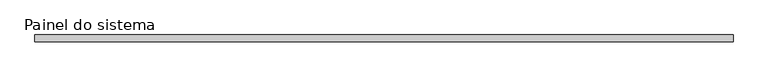
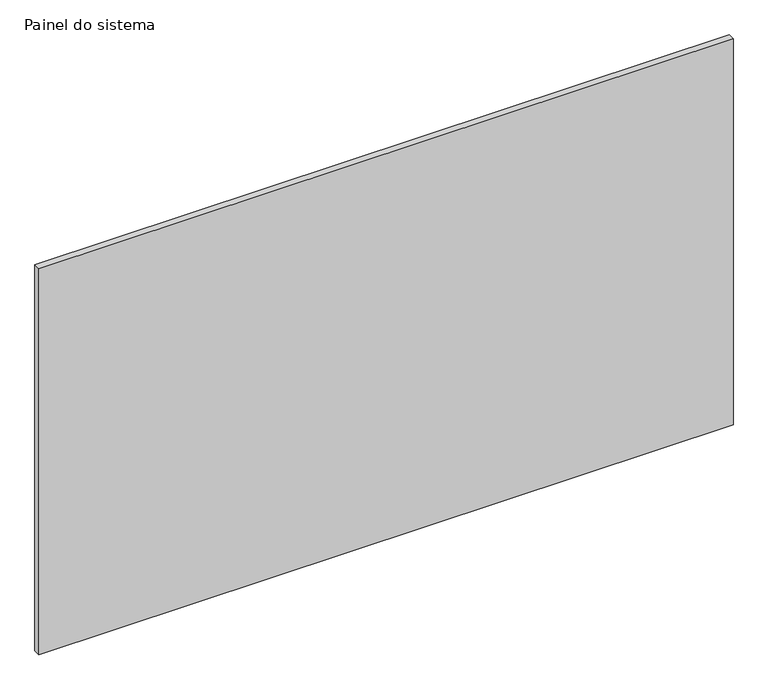
"""IFC4 building model written with IfcOpenShell, lengths in millimetres: plate geometry, Painel do sistema : Envidraçado."""

import ifcopenshell
import ifcopenshell.guid

model = None  # the IFC model being written
_history = None  # IfcOwnerHistory: only IFC2X3 demands one
_inside = {}  # id of a spatial element -> (the spatial element, [elements in it])
_under = {}  # id of a project, library or spatial element -> (it, [spatial elements below it])
_declared = {}  # id of a project -> (the project, [libraries it declares])
_typed = {}  # id of a type object -> (the type object, [elements of that type])
_made_of = {}  # id of a material, layer set ... -> (it, [elements and type objects made of it])


def new_model(schema):
    """Start an empty IFC model of exactly this schema.

    Asked for "IFC4X3", IfcOpenShell would pick the latest addendum, in which some entities
    have other attributes; the version numbers below select the first issue.
    IFC2X3 requires an IfcOwnerHistory on every rooted entity: one is made here for all.
    """
    global model, _history
    if schema == "IFC4X3":
        model = ifcopenshell.file(schema_version=(4, 3, 0, 0))
    else:
        model = ifcopenshell.file(schema=schema)
    _inside.clear()
    _under.clear()
    _declared.clear()
    _typed.clear()
    _made_of.clear()
    _history = None
    if model.schema == "IFC2X3":
        org = make("IfcOrganization", Name="unknown")
        user = make(
            "IfcPersonAndOrganization",
            ThePerson=make("IfcPerson", FamilyName="unknown"),
            TheOrganization=org,
        )
        app = make(
            "IfcApplication",
            ApplicationDeveloper=org,
            Version="unknown",
            ApplicationFullName="unknown",
            ApplicationIdentifier="unknown",
        )
        _history = make(
            "IfcOwnerHistory",
            OwningUser=user,
            OwningApplication=app,
            ChangeAction="ADDED",
            CreationDate=0,
        )
    return model


def make(cls, **values):
    """One entity of the class cls with the attributes given. An attribute that is None is left unset."""
    return model.create_entity(
        cls, **{name: value for name, value in values.items() if value is not None}
    )


def rooted(cls, **values):
    """An entity with a GlobalId (a new one), such as an element, a storey or a relation."""
    return make(cls, GlobalId=ifcopenshell.guid.new(), OwnerHistory=_history, **values)


def si_unit(unit_type, name, prefix=None):
    """IfcSIUnit, for example si_unit("LENGTHUNIT", "METRE", prefix="MILLI")."""
    return make("IfcSIUnit", UnitType=unit_type, Prefix=prefix, Name=name)


def assignment(units):
    """IfcUnitAssignment: the units of a project."""
    return None if units is None else make("IfcUnitAssignment", Units=units)


def point(xyz):
    """IfcCartesianPoint."""
    return None if xyz is None else make("IfcCartesianPoint", Coordinates=xyz)


def direction(xyz):
    """IfcDirection."""
    return None if xyz is None else make("IfcDirection", DirectionRatios=xyz)


def frame(location, z_axis=None, x_axis=None):
    """IfcAxis2Placement3D, a coordinate frame: its origin and axes. An axis left out is left unset."""
    return make(
        "IfcAxis2Placement3D",
        Location=point(location),
        Axis=direction(z_axis),
        RefDirection=direction(x_axis),
    )


def origin():
    """The frame at (0, 0, 0) with its axes left unset."""
    return frame((0.0, 0.0, 0.0))


def origin_with_axes():
    """The frame at (0, 0, 0) with the z axis (0, 0, 1) and the x axis (1, 0, 0) written out."""
    return frame((0.0, 0.0, 0.0), z_axis=(0.0, 0.0, 1.0), x_axis=(1.0, 0.0, 0.0))


def place(relative_to, where):
    """IfcLocalPlacement: puts the frame where relative to a parent placement (None: the world)."""
    return make(
        "IfcLocalPlacement", PlacementRelTo=relative_to, RelativePlacement=where
    )


def context(
    kind, dimensions, precision=None, world=None, true_north=None, identifier=None
):
    """IfcGeometricRepresentationContext, for example the 3D "Model" context."""
    return make(
        "IfcGeometricRepresentationContext",
        ContextIdentifier=identifier,
        ContextType=kind,
        CoordinateSpaceDimension=dimensions,
        Precision=precision,
        WorldCoordinateSystem=world,
        TrueNorth=true_north,
    )


def project(units=None, contexts=None):
    """IfcProject with its units and contexts."""
    return rooted(
        "IfcProject",
        Name="project",
        RepresentationContexts=contexts,
        UnitsInContext=assignment(units),
    )


def spatial(cls, under=None, at=None, **own):
    """A site, building, storey or space (cls), placed at a placement, below another one or the project."""
    s = rooted(cls, ObjectPlacement=at, **own)
    if under is not None:
        _under.setdefault(under.id(), (under, []))[1].append(s)
    return s


def polyline(points):
    """IfcPolyline through the points."""
    return make("IfcPolyline", Points=[point(p) for p in points])


def outline(outer, holes=None, kind="AREA"):
    """IfcArbitraryClosedProfileDef: a profile drawn as a closed curve; with holes, ...WithVoids."""
    if holes is None:
        return make("IfcArbitraryClosedProfileDef", ProfileType=kind, OuterCurve=outer)
    return make(
        "IfcArbitraryProfileDefWithVoids",
        ProfileType=kind,
        OuterCurve=outer,
        InnerCurves=holes,
    )


def extrude(swept, where, along, depth):
    """IfcExtrudedAreaSolid: the profile swept, set in the frame where, extruded along a direction by depth."""
    return make(
        "IfcExtrudedAreaSolid",
        SweptArea=swept,
        Position=where,
        ExtrudedDirection=direction(along),
        Depth=depth,
    )


def shape(context_of_items, identifier, shape_type, items):
    """IfcShapeRepresentation: the items that make up one representation, for example the "Body"."""
    return make(
        "IfcShapeRepresentation",
        ContextOfItems=context_of_items,
        RepresentationIdentifier=identifier,
        RepresentationType=shape_type,
        Items=items,
    )


def source(mapping_origin, context_of_items, identifier, shape_type, items):
    """IfcRepresentationMap: a shape defined once, which mapped items show again and again."""
    return make(
        "IfcRepresentationMap",
        MappingOrigin=mapping_origin,
        MappedRepresentation=shape(context_of_items, identifier, shape_type, items),
    )


def transform(
    local_origin,
    x_axis=None,
    y_axis=None,
    z_axis=None,
    scale=None,
    scale2=None,
    scale3=None,
    uniform=True,
):
    """IfcCartesianTransformationOperator3D, or its non-uniform kind. x_axis, y_axis, z_axis: its Axis1, 2, 3."""
    if uniform:
        return make(
            "IfcCartesianTransformationOperator3D",
            Axis1=direction(x_axis),
            Axis2=direction(y_axis),
            LocalOrigin=point(local_origin),
            Scale=scale,
            Axis3=direction(z_axis),
        )
    return make(
        "IfcCartesianTransformationOperator3DnonUniform",
        Axis1=direction(x_axis),
        Axis2=direction(y_axis),
        LocalOrigin=point(local_origin),
        Scale=scale,
        Axis3=direction(z_axis),
        Scale2=scale2,
        Scale3=scale3,
    )


def mapped(mapping_source, mapping_target):
    """IfcMappedItem: shows the shape of a source again, moved by a transform."""
    return make(
        "IfcMappedItem", MappingSource=mapping_source, MappingTarget=mapping_target
    )


def made_of(thing, what):
    """Note that an element or type object is made of a material, layer set ...; save() writes the relation."""
    if what is not None:
        _made_of.setdefault(what.id(), (what, []))[1].append(thing)
    return thing


def element(
    cls,
    number,
    at=None,
    inside=None,
    cuts=None,
    type_object=None,
    material=None,
    context=None,
    identifier="Body",
    shape_type=None,
    held_by="IfcProductDefinitionShape",
    body=None,
    shapes=None,
    **own,
):
    """One element of the class cls, such as IfcWall. Its Tag is "e" and its number.

    at: its placement. inside: the storey or other place that contains it. cuts: it is an
    opening in that element (IfcRelVoidsElement). A single representation is given by context,
    identifier, shape_type and body (its items); several are given by shapes. held_by: the class
    of the entity that holds the representations. save() writes the other relations.
    """
    e = rooted(cls, Tag="e%d" % number, ObjectPlacement=at, **own)
    if body is not None:
        shapes = [shape(context, identifier, shape_type, body)]
    if shapes is not None:
        e.Representation = make(held_by, Representations=shapes)
    if inside is not None:
        _inside.setdefault(inside.id(), (inside, []))[1].append(e)
    if cuts is not None:
        rooted(
            "IfcRelVoidsElement", RelatingBuildingElement=cuts, RelatedOpeningElement=e
        )
    if type_object is not None:
        _typed.setdefault(type_object.id(), (type_object, []))[1].append(e)
    return made_of(e, material)


def aggregate(whole, parts):
    """IfcRelAggregates: a whole, such as a stair, and the parts it consists of."""
    return rooted("IfcRelAggregates", RelatingObject=whole, RelatedObjects=parts)


def save(model, path):
    """Write the relations noted so far, then the file.

    IfcRelAggregates (storeys below a building ...), IfcRelContainedInSpatialStructure (elements
    in a storey), IfcRelDefinesByType, IfcRelAssociatesMaterial and IfcRelDeclares: one each for
    every whole, place, type object, material and project.
    """
    for whole, parts in _under.values():
        aggregate(whole, parts)
    for where, things in _inside.values():
        rooted(
            "IfcRelContainedInSpatialStructure",
            RelatedElements=things,
            RelatingStructure=where,
        )
    for kind, things in _typed.values():
        rooted("IfcRelDefinesByType", RelatedObjects=things, RelatingType=kind)
    for what, things in _made_of.values():
        rooted("IfcRelAssociatesMaterial", RelatedObjects=things, RelatingMaterial=what)
    for by, libraries in _declared.values():
        rooted("IfcRelDeclares", RelatingContext=by, RelatedDefinitions=libraries)
    model.write(path)


def painel_do_sistema_bfc8fefc(model_context):
    return source(origin(), model_context, "Body", "SweptSolid", [
        extrude(outline(polyline([(1275.8375317, -49.5), (-1275.8375317, -49.5), (-1275.8375317, -24.5), (1275.8375317, -24.5), (1275.8375317, -49.5)])), origin_with_axes(), (0.0, 0.0, 1.0), 1500.0),
    ])


if __name__ == "__main__":
    model = new_model("IFC4")
    model_context = context("Model", 3, world=origin())
    ifc_project = project(units=[si_unit("LENGTHUNIT", "METRE", prefix="MILLI")], contexts=[model_context])
    site = spatial("IfcSite", under=ifc_project)
    building = spatial("IfcBuilding", under=site)
    placement = place(None, origin())
    painel_do_sistema_shape = painel_do_sistema_bfc8fefc(model_context)
    element("IfcPlate", 1, ObjectType="Painel do sistema : Envidraçado", at=placement, inside=building, context=model_context, shape_type="MappedRepresentation", body=[
        mapped(painel_do_sistema_shape, transform((0.0, 0.0, 0.0), x_axis=(1.0, 0.0, 0.0), y_axis=(0.0, 1.0, 0.0), z_axis=(0.0, 0.0, 1.0))),
    ])
    save(model, "model.ifc")

# Revit data of these elements
# Type "Painel do sistema : Envidraçado"
#   Construction Type Id = "GSP4R"
#   Analytic Construction = "Vidraça única Pilkington 1/8 pol"
#   Visual Light Transmittance = 0.9
#   Solar Heat Gain Coefficient = 0.86
#   Heat Transfer Coefficient (U) = 6.7069 W/(m²·K)
# Element 1 (IfcPlate, "Painel do sistema : Envidraçado")
#   Materials on its faces: "Vidro"
# Materials
#   "Vidro": class "Vidro", colour RGB 0 128 192, transparency 0.9, Description = "Vidro de sílica", Cost = 0
